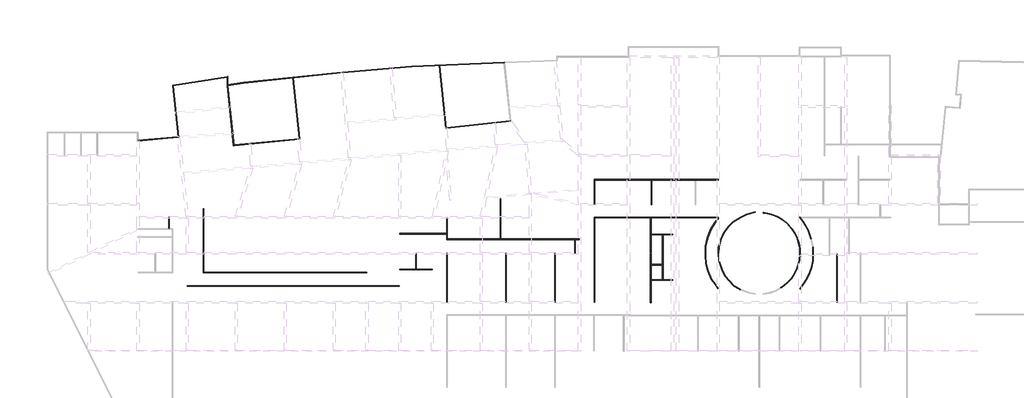
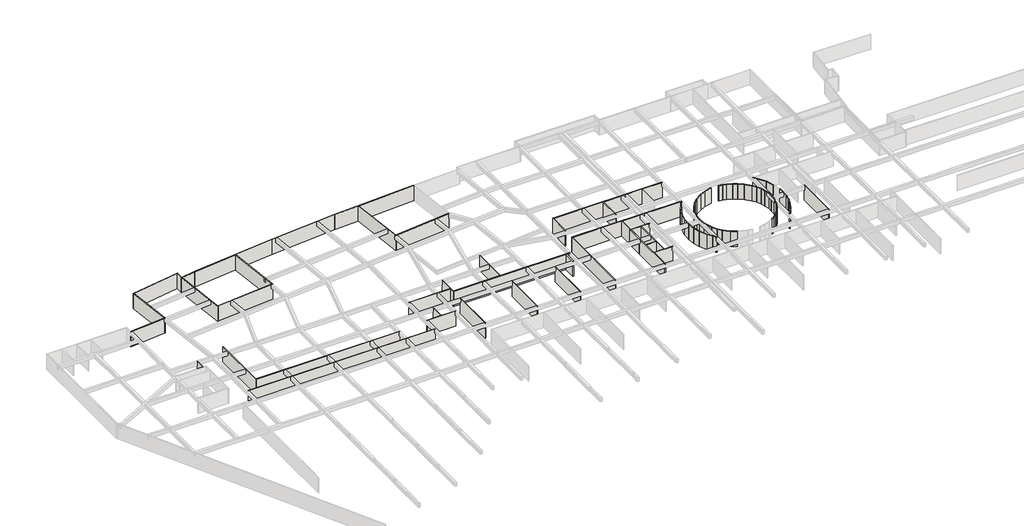
# One storey, part 3 of 8: 90 walls.
"""IFC4 building model written with IfcOpenShell, lengths in millimetres."""

from ifc_helpers import new_model, si_unit, origin, origin_with_axes, place, context, project, spatial, polyline, outline, extrude, faceted_brep, element, save

model = new_model("IFC4")

# Units and contexts
model_context = context("Model", 3, world=origin())
ifc_project = project(units=[si_unit("LENGTHUNIT", "METRE", prefix="MILLI")], contexts=[model_context])

# Site, building, storey
site = spatial("IfcSite", under=ifc_project)
building = spatial("IfcBuilding", under=site)
storey = spatial("IfcBuildingStorey", under=building, Name="户型图", Elevation=0.0)

# Walls
placement = place(None, origin())
element("IfcWall", 1, ObjectType="所有墙体", at=placement, inside=storey, context=model_context, shape_type="Brep", body=[
    faceted_brep([(383558.0584634, 41636.7699948, 0.0), (366573.4477395, 40880.9194972, 0.0), (366573.4477395, 40880.9194972, 3300.0), (383558.0584634, 41636.7699948, 3300.0), (383562.9450973, 41516.8686928, 0.0), (383562.9450973, 41516.8686928, 3300.0), (383506.7284721, 41514.3669361, 3300.0), (371707.7574877, 40989.2881907, 3300.0), (371587.6591107, 40983.9435632, 3300.0), (366581.1732929, 40761.144533, 3300.0), (366581.1732929, 40761.144533, 0.0), (371587.6591107, 40983.9435632, 0.0), (371707.7574877, 40989.2881907, 0.0), (383506.7284721, 41514.3669361, 0.0)], [[[0, 1, 2, 3]], [[4, 5, 6, 7, 8, 9, 10, 11, 12, 13]], [[1, 0, 4, 13, 12, 11, 10]], [[3, 2, 9, 8, 7, 6, 5]], [[0, 3, 5, 4]], [[2, 1, 10, 9]]]),
])
element("IfcWall", 2, ObjectType="所有墙体", at=placement, inside=storey, context=model_context, shape_type="SweptSolid", body=[
    extrude(outline(polyline([(352820.7139757, 39718.1180146), (366573.4477395, 40880.9194972), (366581.1732929, 40761.144533), (352832.0346733, 39598.647022), (352820.7139757, 39718.1180146)])), origin_with_axes(), (0.0, 0.0, 1.0), 3300.0),
])
element("IfcWall", 3, ObjectType="所有墙体", at=placement, inside=storey, context=model_context, shape_type="Brep", body=[
    faceted_brep([(352820.7139757, 39718.1180146, 0.0), (335712.6487947, 37922.0658036, 0.0), (335712.6487947, 37922.0658036, 3300.0), (352820.7139757, 39718.1180146, 3300.0), (352832.0346733, 39598.647022, 0.0), (352832.0346733, 39598.647022, 3300.0), (344839.8399331, 38759.6042149, 3300.0), (344720.4957997, 38747.0751362, 3300.0), (335728.1149338, 37803.0300109, 3300.0), (335728.1149338, 37803.0300109, 0.0), (344720.4957997, 38747.0751362, 0.0), (344839.8399331, 38759.6042149, 0.0)], [[[0, 1, 2, 3]], [[4, 5, 6, 7, 8, 9, 10, 11]], [[1, 0, 4, 11, 10, 9]], [[3, 2, 8, 7, 6, 5]], [[0, 3, 5, 4]], [[2, 1, 9, 8]]]),
])
element("IfcWall", 4, ObjectType="所有墙体", at=placement, inside=storey, context=model_context, shape_type="Brep", body=[
    faceted_brep([(335712.6487947, 37922.0658036, 0.0), (332815.798101, 37472.9548339, 0.0), (332695.798101, 37454.3507282, 0.0), (332695.798101, 37454.3507282, 3300.0), (332815.798101, 37472.9548339, 3300.0), (335712.6487947, 37922.0658036, 3300.0), (335728.1149338, 37803.0300109, 0.0), (335728.1149338, 37803.0300109, 3300.0), (332821.4337723, 37352.3949824, 3300.0), (332702.7066941, 37333.9882231, 3300.0), (332695.798101, 37332.9171548, 3300.0), (332695.798101, 37332.9171548, 0.0), (332702.7066941, 37333.9882231, 0.0), (332821.4337723, 37352.3949824, 0.0)], [[[0, 1, 2, 3, 4, 5]], [[6, 7, 8, 9, 10, 11, 12, 13]], [[2, 1, 0, 6, 13, 12, 11]], [[5, 4, 3, 10, 9, 8, 7]], [[0, 5, 7, 6]], [[3, 2, 11, 10]]]),
])
element("IfcWall", 5, ObjectType="所有墙体", at=placement, inside=storey, context=model_context, shape_type="Brep", body=[
    faceted_brep([(332815.798101, 37472.9548339, 0.0), (332815.798101, 39016.8033625, 0.0), (332815.798101, 39016.8033625, 3300.0), (332815.798101, 37472.9548339, 3300.0), (332695.798101, 37454.3507282, 0.0), (332695.798101, 37454.3507282, 3300.0), (332695.798101, 38876.3141959, 3300.0), (332695.798101, 38997.8082824, 3300.0), (332695.798101, 38997.8082824, 0.0), (332695.798101, 38876.3141959, 0.0)], [[[0, 1, 2, 3]], [[4, 5, 6, 7, 8, 9]], [[1, 0, 4, 9, 8]], [[3, 2, 7, 6, 5]], [[0, 3, 5, 4]], [[2, 1, 8, 7]]]),
])
element("IfcWall", 6, ObjectType="所有墙体", at=placement, inside=storey, context=model_context, shape_type="Brep", body=[
    faceted_brep([(332695.798101, 38997.8082824, 0.0), (322714.3872212, 37417.8274582, 0.0), (322714.3872212, 37417.8274582, 3300.0), (332695.798101, 38997.8082824, 3300.0), (332695.798101, 38876.3141959, 0.0), (332695.798101, 38876.3141959, 3300.0), (322845.6206459, 37317.1066168, 3300.0), (322726.933514, 37298.3193537, 3300.0), (322726.933514, 37298.3193537, 0.0), (322845.6206459, 37317.1066168, 0.0)], [[[0, 1, 2, 3]], [[4, 5, 6, 7, 8, 9]], [[1, 0, 4, 9, 8]], [[3, 2, 7, 6, 5]], [[0, 3, 5, 4]], [[2, 1, 8, 7]]]),
])
element("IfcWall", 7, ObjectType="所有墙体", at=placement, inside=storey, context=model_context, shape_type="Brep", body=[
    faceted_brep([(322726.933514, 37298.3193537, 0.0), (323705.8882933, 27973.4110515, 0.0), (323718.4180279, 27854.0606703, 0.0), (323718.4180279, 27854.0606703, 3300.0), (323705.8882933, 27973.4110515, 3300.0), (322726.933514, 37298.3193537, 3300.0), (322845.6206459, 37317.1066168, 0.0), (322845.6206459, 37317.1066168, 3300.0), (323837.890365, 27865.3685617, 3300.0), (323837.890365, 27865.3685617, 0.0)], [[[0, 1, 2, 3, 4, 5]], [[6, 7, 8, 9]], [[2, 1, 0, 6, 9]], [[5, 4, 3, 8, 7]], [[0, 5, 7, 6]], [[3, 2, 9, 8]]]),
])
element("IfcWall", 8, ObjectType="所有墙体", at=placement, inside=storey, context=model_context, shape_type="Brep", body=[
    faceted_brep([(323705.8882933, 27973.4110515, 0.0), (316365.2591436, 27278.6306619, 0.0), (316245.2591436, 27267.272828, 0.0), (316245.2591436, 27267.272828, 3300.0), (316365.2591436, 27278.6306619, 3300.0), (323705.8882933, 27973.4110515, 3300.0), (323718.4180279, 27854.0606703, 0.0), (323718.4180279, 27854.0606703, 3300.0), (316245.2591436, 27146.7365248, 3300.0), (316245.2591436, 27146.7365248, 0.0)], [[[0, 1, 2, 3, 4, 5]], [[6, 7, 8, 9]], [[2, 1, 0, 6, 9]], [[5, 4, 3, 8, 7]], [[0, 5, 7, 6]], [[3, 2, 9, 8]]]),
])
element("IfcWall", 9, ObjectType="所有墙体", at=placement, inside=storey, context=model_context, shape_type="Brep", body=[
    faceted_brep([(332702.7066941, 37333.9882231, 0.0), (333861.2824935, 26298.1229119, 0.0), (333861.2824935, 26298.1229119, 3300.0), (332702.7066941, 37333.9882231, 3300.0), (332821.4337723, 37352.3949824, 0.0), (332821.4337723, 37352.3949824, 3300.0), (333968.1932646, 26429.0843897, 3300.0), (333980.7227117, 26309.7367468, 3300.0), (333980.7227117, 26309.7367468, 0.0), (333968.1932646, 26429.0843897, 0.0)], [[[0, 1, 2, 3]], [[4, 5, 6, 7, 8, 9]], [[1, 0, 4, 9, 8]], [[3, 2, 7, 6, 5]], [[0, 3, 5, 4]], [[2, 1, 8, 7]]]),
])
element("IfcWall", 10, ObjectType="所有墙体", at=placement, inside=storey, context=model_context, shape_type="Brep", body=[
    faceted_brep([(333980.7227117, 26309.7367468, 0.0), (346023.9239134, 27480.7639956, 0.0), (346023.9239134, 27480.7639956, 3300.0), (333980.7227117, 26309.7367468, 3300.0), (333968.1932646, 26429.0843897, 0.0), (333968.1932646, 26429.0843897, 3300.0), (345891.954248, 27588.4978036, 3300.0), (346011.3944663, 27600.1116384, 3300.0), (346011.3944663, 27600.1116384, 0.0), (345891.954248, 27588.4978036, 0.0)], [[[0, 1, 2, 3]], [[4, 5, 6, 7, 8, 9]], [[1, 0, 4, 9, 8]], [[3, 2, 7, 6, 5]], [[0, 3, 5, 4]], [[2, 1, 8, 7]]]),
])
element("IfcWall", 11, ObjectType="所有墙体", at=placement, inside=storey, context=model_context, shape_type="SweptSolid", body=[
    extrude(outline(polyline([(344839.8399331, 38759.6042149), (346011.3944663, 27600.1116384), (345891.954248, 27588.4978036), (344720.4957997, 38747.0751362), (344839.8399331, 38759.6042149)])), origin_with_axes(), (0.0, 0.0, 1.0), 3300.0),
])
element("IfcWall", 12, ObjectType="所有墙体", at=placement, inside=storey, context=model_context, shape_type="Brep", body=[
    faceted_brep([(371587.6591107, 40983.9435632, 0.0), (372792.8163058, 29504.3731357, 0.0), (372792.8163058, 29504.3731357, 3300.0), (371587.6591107, 40983.9435632, 3300.0), (371707.7574877, 40989.2881907, 0.0), (371707.7574877, 40989.2881907, 3300.0), (372899.6313606, 29636.2463479, 3300.0), (372912.1604393, 29516.9022144, 3300.0), (372912.1604393, 29516.9022144, 0.0), (372899.6313606, 29636.2463479, 0.0)], [[[0, 1, 2, 3]], [[4, 5, 6, 7, 8, 9]], [[1, 0, 4, 9, 8]], [[3, 2, 7, 6, 5]], [[0, 3, 5, 4]], [[2, 1, 8, 7]]]),
])
element("IfcWall", 13, ObjectType="所有墙体", at=placement, inside=storey, context=model_context, shape_type="SweptSolid", body=[
    extrude(outline(polyline([(384637.0313479, 30747.8117356), (372912.1604393, 29516.9022144), (372899.6313606, 29636.2463479), (384624.5022692, 30867.155869), (384637.0313479, 30747.8117356)])), origin_with_axes(), (0.0, 0.0, 1.0), 3300.0),
])
element("IfcWall", 14, ObjectType="所有墙体", at=placement, inside=storey, context=model_context, shape_type="SweptSolid", body=[
    extrude(outline(polyline([(426919.4358549, 13085.7989296), (425600.2025973, 12261.4504989), (425525.0175405, 12355.9710696), (426862.0698044, 13191.4540512), (426919.4358549, 13085.7989296)])), origin_with_axes(), (0.0, 0.0, 1.0), 3300.0),
])
element("IfcWall", 15, ObjectType="所有墙体", at=placement, inside=storey, context=model_context, shape_type="SweptSolid", body=[
    extrude(outline(polyline([(428048.3036822, 13612.1986425), (426919.4358549, 13085.7989296), (426862.0698044, 13191.4540512), (428006.7666734, 13725.2349675), (428048.3036822, 13612.1986425)])), origin_with_axes(), (0.0, 0.0, 1.0), 3300.0),
])
element("IfcWall", 16, ObjectType="所有墙体", at=placement, inside=storey, context=model_context, shape_type="SweptSolid", body=[
    extrude(outline(polyline([(429619.7516013, 14043.6706887), (428048.3036822, 13612.1986425), (428006.7666734, 13725.2349675), (429587.9791139, 14159.3880558), (429619.7516013, 14043.6706887)])), origin_with_axes(), (0.0, 0.0, 1.0), 3300.0),
])
element("IfcWall", 17, ObjectType="所有墙体", at=placement, inside=storey, context=model_context, shape_type="SweptSolid", body=[
    extrude(outline(polyline([(424668.5997813, 11499.5533105), (425525.0175405, 12355.9710696), (425600.2025973, 12261.4504989), (424759.5640815, 11420.8119832), (424668.5997813, 11499.5533105)])), origin_with_axes(), (0.0, 0.0, 1.0), 3300.0),
])
element("IfcWall", 18, ObjectType="所有墙体", at=placement, inside=storey, context=model_context, shape_type="SweptSolid", body=[
    extrude(outline(polyline([(423881.4058067, 10445.7879152), (424668.5997813, 11499.5533105), (424759.5640815, 11420.8119832), (423985.1422552, 10384.1438326), (423881.4058067, 10445.7879152)])), origin_with_axes(), (0.0, 0.0, 1.0), 3300.0),
])
element("IfcWall", 19, ObjectType="所有墙体", at=placement, inside=storey, context=model_context, shape_type="SweptSolid", body=[
    extrude(outline(polyline([(423292.1382111, 9163.4442939), (423881.4058067, 10445.7879152), (423985.1422552, 10384.1438326), (423405.2739104, 9122.2545335), (423292.1382111, 9163.4442939)])), origin_with_axes(), (0.0, 0.0, 1.0), 3300.0),
])
element("IfcWall", 20, ObjectType="所有墙体", at=placement, inside=storey, context=model_context, shape_type="SweptSolid", body=[
    extrude(outline(polyline([(422873.9675555, 7638.0689689), (423292.1382111, 9163.4442939), (423405.2739104, 9122.2545335), (422992.795838, 7617.6442378), (422873.9675555, 7638.0689689)])), origin_with_axes(), (0.0, 0.0, 1.0), 3300.0),
])
element("IfcWall", 21, ObjectType="所有墙体", at=placement, inside=storey, context=model_context, shape_type="SweptSolid", body=[
    extrude(outline(polyline([(422793.6663132, 6538.0871012), (422873.9675555, 7638.0689689), (422992.795838, 7617.6442378), (422914.0644021, 6539.1658796), (422793.6663132, 6538.0871012)])), origin_with_axes(), (0.0, 0.0, 1.0), 3300.0),
])
element("IfcWall", 22, ObjectType="所有墙体", at=placement, inside=storey, context=model_context, shape_type="SweptSolid", body=[
    extrude(outline(polyline([(422918.0331202, 5172.0655357), (422793.6663132, 6538.0871012), (422914.0644021, 6539.1658796), (423036.3186499, 5196.3482654), (422918.0331202, 5172.0655357)])), origin_with_axes(), (0.0, 0.0, 1.0), 3300.0),
])
element("IfcWall", 23, ObjectType="所有墙体", at=placement, inside=storey, context=model_context, shape_type="SweptSolid", body=[
    extrude(outline(polyline([(423534.7757005, 3273.9270497), (422918.0331202, 5172.0655357), (423036.3186499, 5196.3482654), (423645.005003, 3323.0042972), (423534.7757005, 3273.9270497)])), origin_with_axes(), (0.0, 0.0, 1.0), 3300.0),
])
element("IfcWall", 24, ObjectType="所有墙体", at=placement, inside=storey, context=model_context, shape_type="SweptSolid", body=[
    extrude(outline(polyline([(424115.9867993, 2267.2398966), (423534.7757005, 3273.9270497), (423645.005003, 3323.0042972), (424215.6457503, 2334.62553), (424115.9867993, 2267.2398966)])), origin_with_axes(), (0.0, 0.0, 1.0), 3300.0),
])
element("IfcWall", 25, ObjectType="所有墙体", at=placement, inside=storey, context=model_context, shape_type="SweptSolid", body=[
    extrude(outline(polyline([(424722.730959, 1494.2686048), (424115.9867993, 2267.2398966), (424215.6457503, 2334.62553), (424812.6768607, 1574.0283307), (424722.730959, 1494.2686048)])), origin_with_axes(), (0.0, 0.0, 1.0), 3300.0),
])
element("IfcWall", 26, ObjectType="所有墙体", at=placement, inside=storey, context=model_context, shape_type="SweptSolid", body=[
    extrude(outline(polyline([(425720.8125391, 496.1870248), (424722.730959, 1494.2686048), (424812.6768607, 1574.0283307), (425794.494268, 592.2109234), (425720.8125391, 496.1870248)])), origin_with_axes(), (0.0, 0.0, 1.0), 3300.0),
])
element("IfcWall", 27, ObjectType="所有墙体", at=placement, inside=storey, context=model_context, shape_type="SweptSolid", body=[
    extrude(outline(polyline([(426928.370024, -200.9966142), (425720.8125391, 496.1870248), (425794.494268, 592.2109234), (426979.2779354, -91.8242459), (426928.370024, -200.9966142)])), origin_with_axes(), (0.0, 0.0, 1.0), 3300.0),
])
element("IfcWall", 28, ObjectType="所有墙体", at=placement, inside=storey, context=model_context, shape_type="SweptSolid", body=[
    extrude(outline(polyline([(434973.2874621, 553.988382), (434310.2990917, 96.4273342), (434248.2402677, 199.4014838), (434899.7271281, 649.0247709), (434973.2874621, 553.988382)])), origin_with_axes(), (0.0, 0.0, 1.0), 3300.0),
])
element("IfcWall", 29, ObjectType="所有墙体", at=placement, inside=storey, context=model_context, shape_type="SweptSolid", body=[
    extrude(outline(polyline([(435613.1131657, 1107.6347611), (434973.2874621, 553.988382), (434899.7271281, 649.0247709), (435528.9074478, 1193.4596129), (435613.1131657, 1107.6347611)])), origin_with_axes(), (0.0, 0.0, 1.0), 3300.0),
])
element("IfcWall", 30, ObjectType="所有墙体", at=placement, inside=storey, context=model_context, shape_type="SweptSolid", body=[
    extrude(outline(polyline([(436311.4849228, 1884.3155237), (435613.1131657, 1107.6347611), (435528.9074478, 1193.4596129), (436216.6087248, 1958.2734055), (436311.4849228, 1884.3155237)])), origin_with_axes(), (0.0, 0.0, 1.0), 3300.0),
])
element("IfcWall", 31, ObjectType="所有墙体", at=placement, inside=storey, context=model_context, shape_type="SweptSolid", body=[
    extrude(outline(polyline([(436912.807199, 2778.7333921), (436311.4849228, 1884.3155237), (436216.6087248, 1958.2734055), (436807.8146991, 2837.6440997), (436912.807199, 2778.7333921)])), origin_with_axes(), (0.0, 0.0, 1.0), 3300.0),
])
element("IfcWall", 32, ObjectType="所有墙体", at=placement, inside=storey, context=model_context, shape_type="SweptSolid", body=[
    extrude(outline(polyline([(437376.0051237, 3786.7285857), (436912.807199, 2778.7333921), (436807.8146991, 2837.6440997), (437263.2235848, 3828.6890578), (437376.0051237, 3786.7285857)])), origin_with_axes(), (0.0, 0.0, 1.0), 3300.0),
])
element("IfcWall", 33, ObjectType="所有墙体", at=placement, inside=storey, context=model_context, shape_type="SweptSolid", body=[
    extrude(outline(polyline([(437809.4674181, 5284.9982341), (437376.0051237, 3786.7285857), (437263.2235848, 3828.6890578), (437690.9973752, 5307.2962974), (437809.4674181, 5284.9982341)])), origin_with_axes(), (0.0, 0.0, 1.0), 3300.0),
])
element("IfcWall", 34, ObjectType="所有墙体", at=placement, inside=storey, context=model_context, shape_type="SweptSolid", body=[
    extrude(outline(polyline([(437913.8653576, 6435.9108001), (437809.4674181, 5284.9982341), (437690.9973752, 5307.2962974), (437793.8653576, 6441.3421807), (437913.8653576, 6435.9108001)])), origin_with_axes(), (0.0, 0.0, 1.0), 3300.0),
])
element("IfcWall", 35, ObjectType="所有墙体", at=placement, inside=storey, context=model_context, shape_type="SweptSolid", body=[
    extrude(outline(polyline([(437913.8653576, 7345.1889498), (437913.8653576, 6435.9108001), (437793.8653576, 6441.3421807), (437793.8653576, 7332.064031), (437913.8653576, 7345.1889498)])), origin_with_axes(), (0.0, 0.0, 1.0), 3300.0),
])
element("IfcWall", 36, ObjectType="所有墙体", at=placement, inside=storey, context=model_context, shape_type="SweptSolid", body=[
    extrude(outline(polyline([(437674.7771778, 8425.0951891), (437913.8653576, 7345.1889498), (437793.8653576, 7332.064031), (437558.821627, 8393.7024252), (437674.7771778, 8425.0951891)])), origin_with_axes(), (0.0, 0.0, 1.0), 3300.0),
])
element("IfcWall", 37, ObjectType="所有墙体", at=placement, inside=storey, context=model_context, shape_type="SweptSolid", body=[
    extrude(outline(polyline([(437403.0780452, 9270.65638), (437674.7771778, 8425.0951891), (437558.821627, 8393.7024252), (437291.1410542, 9226.7573623), (437403.0780452, 9270.65638)])), origin_with_axes(), (0.0, 0.0, 1.0), 3300.0),
])
element("IfcWall", 38, ObjectType="所有墙体", at=placement, inside=storey, context=model_context, shape_type="SweptSolid", body=[
    extrude(outline(polyline([(436975.9560345, 10186.0220325), (437403.0780452, 9270.65638), (437291.1410542, 9226.7573623), (436870.5656775, 10128.0929163), (436975.9560345, 10186.0220325)])), origin_with_axes(), (0.0, 0.0, 1.0), 3300.0),
])
element("IfcWall", 39, ObjectType="所有墙体", at=placement, inside=storey, context=model_context, shape_type="SweptSolid", body=[
    extrude(outline(polyline([(436445.5313101, 11016.1424874), (436975.9560345, 10186.0220325), (436870.5656775, 10128.0929163), (436349.7365433, 10943.1961682), (436445.5313101, 11016.1424874)])), origin_with_axes(), (0.0, 0.0, 1.0), 3300.0),
])
element("IfcWall", 40, ObjectType="所有墙体", at=placement, inside=storey, context=model_context, shape_type="SweptSolid", body=[
    extrude(outline(polyline([(435443.3146119, 12129.216895), (436445.5313101, 11016.1424874), (436349.7365433, 10943.1961682), (435361.3364652, 12040.9256647), (435443.3146119, 12129.216895)])), origin_with_axes(), (0.0, 0.0, 1.0), 3300.0),
])
element("IfcWall", 41, ObjectType="所有墙体", at=placement, inside=storey, context=model_context, shape_type="SweptSolid", body=[
    extrude(outline(polyline([(434493.6685796, 12864.5970536), (435443.3146119, 12129.216895), (435361.3364652, 12040.9256647), (434426.9653564, 12764.4773363), (434493.6685796, 12864.5970536)])), origin_with_axes(), (0.0, 0.0, 1.0), 3300.0),
])
element("IfcWall", 42, ObjectType="所有墙体", at=placement, inside=storey, context=model_context, shape_type="SweptSolid", body=[
    extrude(outline(polyline([(433666.2223489, 13334.5110428), (434493.6685796, 12864.5970536), (434426.9653564, 12764.4773363), (433614.1896417, 13226.0598106), (433666.2223489, 13334.5110428)])), origin_with_axes(), (0.0, 0.0, 1.0), 3300.0),
])
element("IfcWall", 43, ObjectType="所有墙体", at=placement, inside=storey, context=model_context, shape_type="SweptSolid", body=[
    extrude(outline(polyline([(432609.1058247, 13754.5237479), (433666.2223489, 13334.5110428), (433614.1896417, 13226.0598106), (432571.7477559, 13640.2419999), (432609.1058247, 13754.5237479)])), origin_with_axes(), (0.0, 0.0, 1.0), 3300.0),
])
element("IfcWall", 44, ObjectType="所有墙体", at=placement, inside=storey, context=model_context, shape_type="SweptSolid", body=[
    extrude(outline(polyline([(431889.6215458, 13941.0732158), (432609.1058247, 13754.5237479), (432571.7477559, 13640.2419999), (431865.3939578, 13823.3869678), (431889.6215458, 13941.0732158)])), origin_with_axes(), (0.0, 0.0, 1.0), 3300.0),
])
element("IfcWall", 45, ObjectType="所有墙体", at=placement, inside=storey, context=model_context, shape_type="SweptSolid", body=[
    extrude(outline(polyline([(431112.9718271, 14060.3304084), (431889.6215458, 13941.0732158), (431865.3939578, 13823.3869678), (431094.7588882, 13941.7205907), (431112.9718271, 14060.3304084)])), origin_with_axes(), (0.0, 0.0, 1.0), 3300.0),
])
element("IfcWall", 46, ObjectType="所有墙体", at=placement, inside=storey, context=model_context, shape_type="Brep", body=[
    faceted_brep([(422853.8653576, 13198.6264904, 0.0), (400093.8653576, 13198.6264904, 0.0), (400093.8653576, 13198.6264904, 3300.0), (422853.8653576, 13198.6264904, 3300.0), (422853.8653576, 13078.6264904, 0.0), (422853.8653576, 13078.6264904, 3300.0), (410513.8653575, 13078.6264904, 3300.0), (410393.8653575, 13078.6264904, 3300.0), (400213.8653576, 13078.6264904, 3300.0), (400093.8653576, 13078.6264904, 3300.0), (400093.8653576, 13078.6264904, 0.0), (400213.8653576, 13078.6264904, 0.0), (410393.8653575, 13078.6264904, 0.0), (410513.8653575, 13078.6264904, 0.0)], [[[0, 1, 2, 3]], [[4, 5, 6, 7, 8, 9, 10, 11, 12, 13]], [[1, 0, 4, 13, 12, 11, 10]], [[3, 2, 9, 8, 7, 6, 5]], [[0, 3, 5, 4]], [[2, 1, 10, 9]]]),
])
element("IfcWall", 47, ObjectType="所有墙体", at=placement, inside=storey, context=model_context, shape_type="SweptSolid", body=[
    extrude(outline(polyline([(400093.8653576, -2461.3735096), (400093.8653576, 13078.6264904), (400213.8653576, 13078.6264904), (400213.8653576, -2461.3735096), (400093.8653576, -2461.3735096)])), origin_with_axes(), (0.0, 0.0, 1.0), 3300.0),
])
element("IfcWall", 48, ObjectType="所有墙体", at=placement, inside=storey, context=model_context, shape_type="SweptSolid", body=[
    extrude(outline(polyline([(410393.8653575, 6638.6264682), (410393.8653575, 13078.6264904), (410513.8653575, 13078.6264904), (410513.8653575, 6638.6264682), (410393.8653575, 6638.6264682)])), origin_with_axes(), (0.0, 0.0, 1.0), 3300.0),
])
element("IfcWall", 49, ObjectType="所有墙体", at=placement, inside=storey, context=model_context, shape_type="Brep", body=[
    faceted_brep([(410513.8653575, 6638.6264682, 0.0), (410513.8653575, 9928.6264684, 0.0), (410513.8653575, 10048.6264684, 0.0), (410513.8653575, 10048.6264684, 3300.0), (410513.8653575, 9928.6264684, 3300.0), (410513.8653575, 6638.6264682, 3300.0), (410393.8653575, 6638.6264682, 0.0), (410393.8653575, 6638.6264682, 3300.0), (410393.8653575, 10048.6264684, 3300.0), (410393.8653575, 10048.6264684, 0.0)], [[[0, 1, 2, 3, 4, 5]], [[6, 7, 8, 9]], [[2, 1, 0, 6, 9]], [[5, 4, 3, 8, 7]], [[0, 5, 7, 6]], [[3, 2, 9, 8]]]),
])
element("IfcWall", 50, ObjectType="所有墙体", at=placement, inside=storey, context=model_context, shape_type="Brep", body=[
    faceted_brep([(414453.8653574, 10048.6264684, 0.0), (410513.8653575, 10048.6264684, 0.0), (410513.8653575, 10048.6264684, 3300.0), (414453.8653574, 10048.6264684, 3300.0), (414453.8653574, 9928.6264684, 0.0), (414453.8653574, 9928.6264684, 3300.0), (412713.8653576, 9928.6264684, 3300.0), (412593.8653576, 9928.6264684, 3300.0), (410513.8653575, 9928.6264684, 3300.0), (410513.8653575, 9928.6264684, 0.0), (412593.8653576, 9928.6264684, 0.0), (412713.8653576, 9928.6264684, 0.0)], [[[0, 1, 2, 3]], [[4, 5, 6, 7, 8, 9, 10, 11]], [[1, 0, 4, 11, 10, 9]], [[3, 2, 8, 7, 6, 5]], [[0, 3, 5, 4]], [[2, 1, 9, 8]]]),
])
element("IfcWall", 51, ObjectType="所有墙体", at=placement, inside=storey, context=model_context, shape_type="Brep", body=[
    faceted_brep([(410393.8653575, 6438.6264682, 0.0), (410393.8653575, -2561.3735318, 0.0), (410393.8653575, -2561.3735318, 3300.0), (410393.8653575, 6438.6264682, 3300.0), (410513.8653575, 6438.6264682, 0.0), (410513.8653575, 6438.6264682, 3300.0), (410513.8653575, 4498.6264778, 3300.0), (410513.8653575, 4378.6264778, 3300.0), (410513.8653575, 1698.6264778, 3300.0), (410513.8653575, 1578.6264778, 3300.0), (410513.8653575, -2561.3735318, 3300.0), (410513.8653575, -2561.3735318, 0.0), (410513.8653575, 1578.6264778, 0.0), (410513.8653575, 1698.6264778, 0.0), (410513.8653575, 4378.6264778, 0.0), (410513.8653575, 4498.6264778, 0.0)], [[[0, 1, 2, 3]], [[4, 5, 6, 7, 8, 9, 10, 11, 12, 13, 14, 15]], [[1, 0, 4, 15, 14, 13, 12, 11]], [[2, 1, 11, 10]], [[3, 2, 10, 9, 8, 7, 6, 5]], [[0, 3, 5, 4]]]),
])
element("IfcWall", 52, ObjectType="所有墙体", at=placement, inside=storey, context=model_context, shape_type="SweptSolid", body=[
    extrude(outline(polyline([(412593.8653576, 4378.6264778), (410513.8653575, 4378.6264778), (410513.8653575, 4498.6264778), (412593.8653576, 4498.6264778), (412593.8653576, 4378.6264778)])), origin_with_axes(), (0.0, 0.0, 1.0), 3300.0),
])
element("IfcWall", 53, ObjectType="所有墙体", at=placement, inside=storey, context=model_context, shape_type="Brep", body=[
    faceted_brep([(412593.8653576, 9928.6264684, 0.0), (412593.8653576, 4498.6264778, 0.0), (412593.8653576, 4378.6264778, 0.0), (412593.8653576, 1698.6264778, 0.0), (412593.8653576, 1698.6264778, 3300.0), (412593.8653576, 4378.6264778, 3300.0), (412593.8653576, 4498.6264778, 3300.0), (412593.8653576, 9928.6264684, 3300.0), (412713.8653576, 9928.6264684, 0.0), (412713.8653576, 9928.6264684, 3300.0), (412713.8653576, 1698.6264778, 3300.0), (412713.8653576, 1698.6264778, 0.0)], [[[0, 1, 2, 3, 4, 5, 6, 7]], [[8, 9, 10, 11]], [[3, 2, 1, 0, 8, 11]], [[7, 6, 5, 4, 10, 9]], [[4, 3, 11, 10]], [[0, 7, 9, 8]]]),
])
element("IfcWall", 54, ObjectType="所有墙体", at=placement, inside=storey, context=model_context, shape_type="Brep", body=[
    faceted_brep([(410513.8653575, 1578.6264778, 0.0), (414453.8653576, 1578.6264778, 0.0), (414453.8653576, 1578.6264778, 3300.0), (410513.8653575, 1578.6264778, 3300.0), (410513.8653575, 1698.6264778, 0.0), (410513.8653575, 1698.6264778, 3300.0), (412593.8653576, 1698.6264778, 3300.0), (412713.8653576, 1698.6264778, 3300.0), (414453.8653576, 1698.6264778, 3300.0), (414453.8653576, 1698.6264778, 0.0), (412713.8653576, 1698.6264778, 0.0), (412593.8653576, 1698.6264778, 0.0)], [[[0, 1, 2, 3]], [[4, 5, 6, 7, 8, 9, 10, 11]], [[1, 0, 4, 11, 10, 9]], [[2, 1, 9, 8]], [[3, 2, 8, 7, 6, 5]], [[0, 3, 5, 4]]]),
])
element("IfcWall", 55, ObjectType="所有墙体", at=placement, inside=storey, context=model_context, shape_type="SweptSolid", body=[
    extrude(outline(polyline([(422145.6178999, 12152.9940943), (422805.7969097, 13036.7328139), (422901.9338055, 12964.9157041), (422245.4658018, 12086.1446671), (422145.6178999, 12152.9940943)])), origin_with_axes(), (0.0, 0.0, 1.0), 3300.0),
])
element("IfcWall", 56, ObjectType="所有墙体", at=placement, inside=storey, context=model_context, shape_type="SweptSolid", body=[
    extrude(outline(polyline([(421408.1396297, 10918.0588563), (422145.6178999, 12152.9940943), (422245.4658018, 12086.1446671), (421516.1039766, 10864.8007229), (421408.1396297, 10918.0588563)])), origin_with_axes(), (0.0, 0.0, 1.0), 3300.0),
])
element("IfcWall", 57, ObjectType="所有墙体", at=placement, inside=storey, context=model_context, shape_type="SweptSolid", body=[
    extrude(outline(polyline([(420842.2560938, 9493.8047104), (421408.1396297, 10918.0588563), (421516.1039766, 10864.8007229), (420956.5378418, 9456.4466416), (420842.2560938, 9493.8047104)])), origin_with_axes(), (0.0, 0.0, 1.0), 3300.0),
])
element("IfcWall", 58, ObjectType="所有墙体", at=placement, inside=storey, context=model_context, shape_type="SweptSolid", body=[
    extrude(outline(polyline([(420412.7259221, 7837.1920738), (420842.2560938, 9493.8047104), (420956.5378418, 9456.4466416), (420532.7259221, 7821.8881682), (420412.7259221, 7837.1920738)])), origin_with_axes(), (0.0, 0.0, 1.0), 3300.0),
])
element("IfcWall", 59, ObjectType="所有墙体", at=placement, inside=storey, context=model_context, shape_type="SweptSolid", body=[
    extrude(outline(polyline([(420412.7259221, 6126.8144652), (420412.7259221, 7837.1920738), (420532.7259221, 7821.8881682), (420532.7259221, 6132.2657769), (420412.7259221, 6126.8144652)])), origin_with_axes(), (0.0, 0.0, 1.0), 3300.0),
])
element("IfcWall", 60, ObjectType="所有墙体", at=placement, inside=storey, context=model_context, shape_type="SweptSolid", body=[
    extrude(outline(polyline([(420549.462666, 4624.9238437), (420412.7259221, 6126.8144652), (420532.7259221, 6132.2657769), (420667.9934363, 4646.5128983), (420549.462666, 4624.9238437)])), origin_with_axes(), (0.0, 0.0, 1.0), 3300.0),
])
element("IfcWall", 61, ObjectType="所有墙体", at=placement, inside=storey, context=model_context, shape_type="SweptSolid", body=[
    extrude(outline(polyline([(420925.2765836, 3264.5485316), (420549.462666, 4624.9238437), (420667.9934363, 4646.5128983), (421038.8740387, 3303.995254), (420925.2765836, 3264.5485316)])), origin_with_axes(), (0.0, 0.0, 1.0), 3300.0),
])
element("IfcWall", 62, ObjectType="所有墙体", at=placement, inside=storey, context=model_context, shape_type="SweptSolid", body=[
    extrude(outline(polyline([(421574.7857714, 1723.6377662), (420925.2765836, 3264.5485316), (421038.8740387, 3303.995254), (421679.1141077, 1785.0747626), (421574.7857714, 1723.6377662)])), origin_with_axes(), (0.0, 0.0, 1.0), 3300.0),
])
element("IfcWall", 63, ObjectType="所有墙体", at=placement, inside=storey, context=model_context, shape_type="SweptSolid", body=[
    extrude(outline(polyline([(422318.0604435, 776.7312749), (421574.7857714, 1723.6377662), (421679.1141077, 1785.0747626), (422417.7193945, 844.1169083), (422318.0604435, 776.7312749)])), origin_with_axes(), (0.0, 0.0, 1.0), 3300.0),
])
element("IfcWall", 64, ObjectType="所有墙体", at=placement, inside=storey, context=model_context, shape_type="SweptSolid", body=[
    extrude(outline(polyline([(422715.9283947, 87.6037685), (422318.0604435, 776.7312749), (422417.7193945, 844.1169083), (422819.8514432, 147.6037685), (422715.9283947, 87.6037685)])), origin_with_axes(), (0.0, 0.0, 1.0), 3300.0),
])
element("IfcWall", 65, ObjectType="所有墙体", at=placement, inside=storey, context=model_context, shape_type="Brep", body=[
    faceted_brep([(437741.8951901, 13198.6264904, 0.0), (438311.2052799, 12342.7221597, 0.0), (438311.2052799, 12342.7221597, 3300.0), (437741.8951901, 13198.6264904, 3300.0), (437886.0167787, 13198.6264904, 0.0), (437886.0167787, 13198.6264904, 3300.0), (437965.8355251, 13078.6264904, 3300.0), (438411.731421, 12408.2638267, 3300.0), (438411.731421, 12408.2638267, 0.0), (437965.8355251, 13078.6264904, 0.0)], [[[0, 1, 2, 3]], [[4, 5, 6, 7, 8, 9]], [[1, 0, 4, 9, 8]], [[3, 2, 7, 6, 5]], [[2, 1, 8, 7]], [[0, 3, 5, 4]]]),
])
element("IfcWall", 66, ObjectType="所有墙体", at=placement, inside=storey, context=model_context, shape_type="SweptSolid", body=[
    extrude(outline(polyline([(439275.9144672, 10832.9418036), (438311.2052799, 12342.7221597), (438411.731421, 12408.2638267), (439385.4052589, 10884.453695), (439275.9144672, 10832.9418036)])), origin_with_axes(), (0.0, 0.0, 1.0), 3300.0),
])
element("IfcWall", 67, ObjectType="所有墙体", at=placement, inside=storey, context=model_context, shape_type="SweptSolid", body=[
    extrude(outline(polyline([(439792.7443416, 9224.5035292), (439275.9144672, 10832.9418036), (439385.4052589, 10884.453695), (439908.6998925, 9255.8962932), (439792.7443416, 9224.5035292)])), origin_with_axes(), (0.0, 0.0, 1.0), 3300.0),
])
element("IfcWall", 68, ObjectType="所有墙体", at=placement, inside=storey, context=model_context, shape_type="SweptSolid", body=[
    extrude(outline(polyline([(440147.6903543, 5191.7488938), (440147.6903543, 7621.2941439), (440267.6903543, 7634.4190627), (440267.6903543, 5179.1363855), (440147.6903543, 5191.7488938)])), origin_with_axes(), (0.0, 0.0, 1.0), 3300.0),
])
element("IfcWall", 69, ObjectType="所有墙体", at=placement, inside=storey, context=model_context, shape_type="SweptSolid", body=[
    extrude(outline(polyline([(439879.6135693, 3930.5467796), (440147.6903543, 5191.7488938), (440267.6903543, 5179.1363855), (439995.1967431, 3897.1547378), (439879.6135693, 3930.5467796)])), origin_with_axes(), (0.0, 0.0, 1.0), 3300.0),
])
element("IfcWall", 70, ObjectType="所有墙体", at=placement, inside=storey, context=model_context, shape_type="SweptSolid", body=[
    extrude(outline(polyline([(439419.4468647, 2681.7385347), (439879.6135693, 3930.5467796), (439995.1967431, 3897.1547378), (439530.0027368, 2634.7033157), (439419.4468647, 2681.7385347)])), origin_with_axes(), (0.0, 0.0, 1.0), 3300.0),
])
element("IfcWall", 71, ObjectType="所有墙体", at=placement, inside=storey, context=model_context, shape_type="SweptSolid", body=[
    extrude(outline(polyline([(438924.6154546, 1661.1281627), (439419.4468647, 2681.7385347), (439530.0027368, 2634.7033157), (439028.9110568, 1601.1808766), (438924.6154546, 1661.1281627)])), origin_with_axes(), (0.0, 0.0, 1.0), 3300.0),
])
element("IfcWall", 72, ObjectType="所有墙体", at=placement, inside=storey, context=model_context, shape_type="SweptSolid", body=[
    extrude(outline(polyline([(437821.5439633, 20.3992371), (438924.6154546, 1661.1281627), (439028.9110568, 1601.1808766), (437921.1300535, -46.553064), (437821.5439633, 20.3992371)])), origin_with_axes(), (0.0, 0.0, 1.0), 3300.0),
])
element("IfcWall", 73, ObjectType="所有墙体", at=placement, inside=storey, context=model_context, shape_type="SweptSolid", body=[
    extrude(outline(polyline([(444593.8653577, -2461.3735096), (444593.8653577, 6438.6264904), (444713.8653577, 6438.6264904), (444713.8653577, -2461.3735096), (444593.8653577, -2461.3735096)])), origin_with_axes(), (0.0, 0.0, 1.0), 3300.0),
])
element("IfcWall", 74, ObjectType="所有墙体", at=placement, inside=storey, context=model_context, shape_type="SweptSolid", body=[
    extrude(outline(polyline([(392793.8653576, -2461.3735096), (392793.8653576, 6538.6264904), (392913.8653576, 6538.6264904), (392913.8653576, -2461.3735096), (392793.8653576, -2461.3735096)])), origin_with_axes(), (0.0, 0.0, 1.0), 3300.0),
])
element("IfcWall", 75, ObjectType="所有墙体", at=placement, inside=storey, context=model_context, shape_type="SweptSolid", body=[
    extrude(outline(polyline([(383793.8653576, -2561.3735094), (383793.8653576, 6538.6264904), (383913.8653576, 6538.6264904), (383913.8653576, -2561.3735094), (383793.8653576, -2561.3735094)])), origin_with_axes(), (0.0, 0.0, 1.0), 3300.0),
])
element("IfcWall", 76, ObjectType="所有墙体", at=placement, inside=storey, context=model_context, shape_type="SweptSolid", body=[
    extrude(outline(polyline([(372993.8653577, -2461.3735096), (372993.8653577, 6538.6264904), (373113.8653577, 6538.6264904), (373113.8653577, -2461.3735096), (372993.8653577, -2461.3735096)])), origin_with_axes(), (0.0, 0.0, 1.0), 3300.0),
])
element("IfcWall", 77, ObjectType="所有墙体", at=placement, inside=storey, context=model_context, shape_type="Brep", body=[
    faceted_brep([(364349.4818595, 3528.6264772, 0.0), (370349.4818595, 3528.6264772, 0.0), (370349.4818595, 3528.6264772, 3300.0), (364349.4818595, 3528.6264772, 3300.0), (364349.4818595, 3648.6264772, 0.0), (364349.4818595, 3648.6264772, 3300.0), (367289.4818595, 3648.6264772, 3300.0), (367409.4818595, 3648.6264772, 3300.0), (370349.4818595, 3648.6264772, 3300.0), (370349.4818595, 3648.6264772, 0.0), (367409.4818595, 3648.6264772, 0.0), (367289.4818595, 3648.6264772, 0.0)], [[[0, 1, 2, 3]], [[4, 5, 6, 7, 8, 9, 10, 11]], [[1, 0, 4, 11, 10, 9]], [[2, 1, 9, 8]], [[3, 2, 8, 7, 6, 5]], [[0, 3, 5, 4]]]),
])
element("IfcWall", 78, ObjectType="所有墙体", at=placement, inside=storey, context=model_context, shape_type="SweptSolid", body=[
    extrude(outline(polyline([(367409.4818595, 6438.6264772), (367409.4818595, 3648.6264772), (367289.4818595, 3648.6264772), (367289.4818595, 6438.6264772), (367409.4818595, 6438.6264772)])), origin_with_axes(), (0.0, 0.0, 1.0), 3300.0),
])
element("IfcWall", 79, ObjectType="所有墙体", at=placement, inside=storey, context=model_context, shape_type="SweptSolid", body=[
    extrude(outline(polyline([(372993.8653576, 10078.6264904), (364353.8653576, 10078.6264904), (364353.8653576, 10198.6264904), (372993.8653576, 10198.6264904), (372993.8653576, 10078.6264904)])), origin_with_axes(), (0.0, 0.0, 1.0), 3300.0),
])
element("IfcWall", 80, ObjectType="所有墙体", at=placement, inside=storey, context=model_context, shape_type="Brep", body=[
    faceted_brep([(373113.8653576, 9078.6264904, 0.0), (373113.8653576, 9198.6264904, 0.0), (373113.8653576, 13038.6264824, 0.0), (373113.8653576, 13038.6264824, 3300.0), (373113.8653576, 9198.6264904, 3300.0), (373113.8653576, 9078.6264904, 3300.0), (372993.8653576, 9078.6264904, 0.0), (372993.8653576, 9078.6264904, 3300.0), (372993.8653576, 10078.6264904, 3300.0), (372993.8653576, 10198.6264904, 3300.0), (372993.8653576, 13038.6264824, 3300.0), (372993.8653576, 13038.6264824, 0.0), (372993.8653576, 10198.6264904, 0.0), (372993.8653576, 10078.6264904, 0.0)], [[[0, 1, 2, 3, 4, 5]], [[6, 7, 8, 9, 10, 11, 12, 13]], [[2, 1, 0, 6, 13, 12, 11]], [[3, 2, 11, 10]], [[5, 4, 3, 10, 9, 8, 7]], [[0, 5, 7, 6]]]),
])
element("IfcWall", 81, ObjectType="所有墙体", at=placement, inside=storey, context=model_context, shape_type="Brep", body=[
    faceted_brep([(373113.8653576, 9078.6264904, 0.0), (396493.8653576, 9078.6264904, 0.0), (396613.8653576, 9078.6264904, 0.0), (397353.8653576, 9078.6264904, 0.0), (397353.8653576, 9078.6264904, 3300.0), (396613.8653576, 9078.6264904, 3300.0), (396493.8653576, 9078.6264904, 3300.0), (373113.8653576, 9078.6264904, 3300.0), (373113.8653576, 9198.6264904, 0.0), (373113.8653576, 9198.6264904, 3300.0), (382793.8653576, 9198.6264904, 3300.0), (382913.8653576, 9198.6264904, 3300.0), (397353.8653576, 9198.6264904, 3300.0), (397353.8653576, 9198.6264904, 0.0), (382913.8653576, 9198.6264904, 0.0), (382793.8653576, 9198.6264904, 0.0)], [[[0, 1, 2, 3, 4, 5, 6, 7]], [[8, 9, 10, 11, 12, 13, 14, 15]], [[3, 2, 1, 0, 8, 15, 14, 13]], [[4, 3, 13, 12]], [[7, 6, 5, 4, 12, 11, 10, 9]], [[0, 7, 9, 8]]]),
])
element("IfcWall", 82, ObjectType="所有墙体", at=placement, inside=storey, context=model_context, shape_type="SweptSolid", body=[
    extrude(outline(polyline([(396493.8653576, 6538.6264904), (396493.8653576, 9078.6264904), (396613.8653576, 9078.6264904), (396613.8653576, 6538.6264904), (396493.8653576, 6538.6264904)])), origin_with_axes(), (0.0, 0.0, 1.0), 3300.0),
])
element("IfcWall", 83, ObjectType="所有墙体", at=placement, inside=storey, context=model_context, shape_type="SweptSolid", body=[
    extrude(outline(polyline([(382913.8653576, 16542.6356509), (382913.8653576, 9198.6264904), (382793.8653576, 9198.6264904), (382793.8653576, 16542.6356509), (382913.8653576, 16542.6356509)])), origin_with_axes(), (0.0, 0.0, 1.0), 3300.0),
])
element("IfcWall", 84, ObjectType="所有墙体", at=placement, inside=storey, context=model_context, shape_type="SweptSolid", body=[
    extrude(outline(polyline([(325353.8653594, 598.6264904), (364253.8653576, 598.6264904), (364253.8653576, 478.6264904), (325353.8653594, 478.6264904), (325353.8653594, 598.6264904)])), origin_with_axes(), (0.0, 0.0, 1.0), 3300.0),
])
element("IfcWall", 85, ObjectType="所有墙体", at=placement, inside=storey, context=model_context, shape_type="Brep", body=[
    faceted_brep([(328293.8653576, 14738.6264904, 0.0), (328293.8653576, 2978.6264904, 0.0), (328293.8653576, 2978.6264904, 3300.0), (328293.8653576, 14738.6264904, 3300.0), (328413.8653576, 14738.6264904, 0.0), (328413.8653576, 14738.6264904, 3300.0), (328413.8653576, 3098.6264904, 3300.0), (328413.8653576, 2978.6264904, 3300.0), (328413.8653576, 2978.6264904, 0.0), (328413.8653576, 3098.6264904, 0.0)], [[[0, 1, 2, 3]], [[4, 5, 6, 7, 8, 9]], [[1, 0, 4, 9, 8]], [[3, 2, 7, 6, 5]], [[0, 3, 5, 4]], [[2, 1, 8, 7]]]),
])
element("IfcWall", 86, ObjectType="所有墙体", at=placement, inside=storey, context=model_context, shape_type="SweptSolid", body=[
    extrude(outline(polyline([(358353.8653576, 2978.6264904), (328413.8653576, 2978.6264904), (328413.8653576, 3098.6264904), (358353.8653576, 3098.6264904), (358353.8653576, 2978.6264904)])), origin_with_axes(), (0.0, 0.0, 1.0), 3300.0),
])
element("IfcWall", 87, ObjectType="所有墙体", at=placement, inside=storey, context=model_context, shape_type="SweptSolid", body=[
    extrude(outline(polyline([(321993.8653557, 11098.6229613), (321993.8653557, 13138.6264904), (322113.8653557, 13138.6264904), (322113.8653557, 11098.6236028), (321993.8653557, 11098.6229613)])), origin_with_axes(), (0.0, 0.0, 1.0), 3300.0),
])
element("IfcWall", 88, ObjectType="所有墙体", at=placement, inside=storey, context=model_context, shape_type="Brep", body=[
    faceted_brep([(400213.8653576, 15538.6264904, 0.0), (400213.8653576, 19978.6264904, 0.0), (400213.8653576, 20098.6264904, 0.0), (400213.8653576, 20098.6264904, 3300.0), (400213.8653576, 19978.6264904, 3300.0), (400213.8653576, 15538.6264904, 3300.0), (400093.8653576, 15538.6264904, 0.0), (400093.8653576, 15538.6264904, 3300.0), (400093.8653576, 20098.6264904, 3300.0), (400093.8653576, 20098.6264904, 0.0)], [[[0, 1, 2, 3, 4, 5]], [[6, 7, 8, 9]], [[2, 1, 0, 6, 9]], [[5, 4, 3, 8, 7]], [[0, 5, 7, 6]], [[3, 2, 9, 8]]]),
])
element("IfcWall", 89, ObjectType="所有墙体", at=placement, inside=storey, context=model_context, shape_type="Brep", body=[
    faceted_brep([(400213.8653576, 19978.6264904, 0.0), (410493.8653576, 19978.6264904, 0.0), (410613.8653576, 19978.6264904, 0.0), (418593.8653576, 19978.6264904, 0.0), (418713.8653576, 19978.6264904, 0.0), (422853.8653576, 19978.6264904, 0.0), (422853.8653576, 19978.6264904, 3300.0), (418713.8653576, 19978.6264904, 3300.0), (418593.8653576, 19978.6264904, 3300.0), (410613.8653576, 19978.6264904, 3300.0), (410493.8653576, 19978.6264904, 3300.0), (400213.8653576, 19978.6264904, 3300.0), (400213.8653576, 20098.6264904, 0.0), (400213.8653576, 20098.6264904, 3300.0), (422853.8653576, 20098.6264904, 3300.0), (422853.8653576, 20098.6264904, 0.0)], [[[0, 1, 2, 3, 4, 5, 6, 7, 8, 9, 10, 11]], [[12, 13, 14, 15]], [[5, 4, 3, 2, 1, 0, 12, 15]], [[6, 5, 15, 14]], [[11, 10, 9, 8, 7, 6, 14, 13]], [[0, 11, 13, 12]]]),
])
element("IfcWall", 90, ObjectType="所有墙体", at=placement, inside=storey, context=model_context, shape_type="SweptSolid", body=[
    extrude(outline(polyline([(410493.8653576, 15438.6264908), (410493.8653576, 19978.6264904), (410613.8653576, 19978.6264904), (410613.8653576, 15438.6264908), (410493.8653576, 15438.6264908)])), origin_with_axes(), (0.0, 0.0, 1.0), 3300.0),
])

save(model, "model.ifc")

# Revit data of these elements
# Type "所有墙体"
#   Layers, outside or top first: 120 mm "默认" (function 1)
# Elements 1, 2, 3, 4, 5, 6, 7, 8, 9, 10, 11, 12, 13, 14, 15, 16, 17, 18, 19, 20, 21, 22, 23, 24, 25, 26, 27, 28, 29, 30, 31, 32, 33, 34, 35, 36, 37, 38, 39, 40, 41, 42, 43, 44, 45, 46, 47, 48, 49, 50, 51, 52, 53, 54, 55, 56, 57, 58, 59, 60, 61, 62, 63, 64, 65, 66, 67, 68, 69, 70, 71, 72, 73, 74, 75, 76, 77, 78, 79, 80, 81, 82, 83, 84, 85, 86, 87, 88, 89, 90 (IfcWall, "所有墙体")
#   Top Offset = 0 mm
#   Base Offset = 0 mm
#   wall height = 3300 mm
#   Phase Created = 新构造
#   Base Constraint = 户型图
#   Top Constraint = 层高
#   Materials on its faces: "默认"
# Materials
#   "默认": class "其他", colour RGB 192 192 192, transparency 0, Cost = 0
